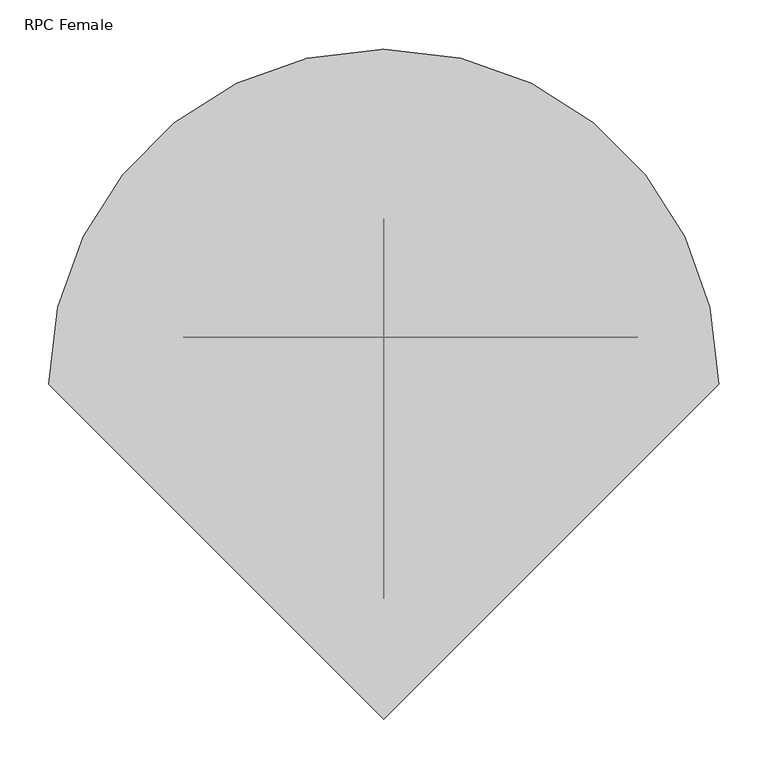
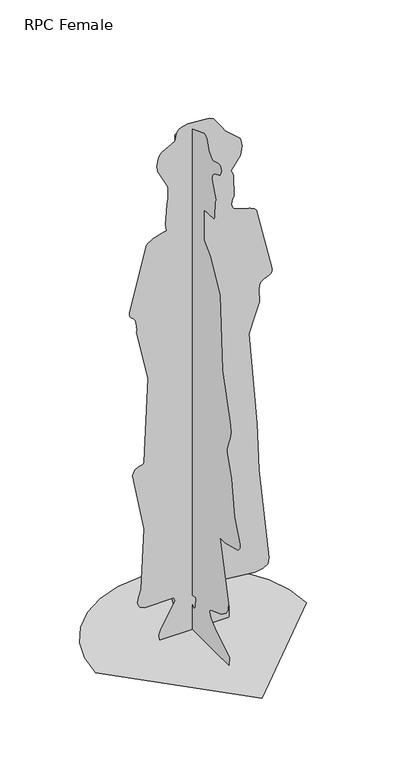
"""IFC4 building model written with IfcOpenShell, lengths in millimetres: proxy geometry, RPC Female : Tina."""

from ifc_helpers import new_model, si_unit, origin, place, context, project, spatial, triangles, source, transform, mapped, element, save


def rpc_female_936a91ee(model_context):
    return source(origin(), model_context, "Body", "Tessellation", [
        triangles([(119.4746024, 47.9851797, 38.3657269), (83.0886148, 47.9851797, 124.5051729), (83.0138374, 47.9851797, 136.8061299), (203.3585538, 47.9851751, 124.5967734), (228.5680434, 47.9851706, 128.329131), (244.5854705, 47.9851706, 139.121441), (247.7915793, 47.9851706, 159.148825), (216.0390116, 47.9851751, 471.099733), (209.7903923, 47.9851751, 633.4228918), (183.5555111, 47.9851751, 949.5239462), (203.8698598, 47.9851751, 1005.6493721), (217.070017, 47.9851751, 1047.2735756), (217.4083866, 47.9851706, 1056.0226055), (217.0055224, 47.9851751, 1064.6613224), (216.3185004, 47.9851751, 1073.2607248), (215.8053413, 47.9851751, 1081.8947908), (215.9203052, 47.9851751, 1090.6344463), (217.1204863, 47.9851751, 1099.5507626), (219.8629788, 47.9851706, 1108.7167002), (224.4103938, 47.9851706, 1115.2149227), (231.1179786, 47.9851706, 1119.4220787), (238.8976818, 47.9851706, 1122.5300285), (246.6605618, 47.9851706, 1125.7305599), (253.3176591, 47.9851706, 1130.2172047), (257.7819034, 47.9851706, 1137.1818232), (258.9624636, 47.9851706, 1147.8162031), (208.6911498, 47.9851751, 1362.8652134), (200.9254719, 47.9851751, 1370.8879795), (188.863799, 47.9851751, 1376.7655277), (174.3222992, 47.9851751, 1381.3783276), (159.1180856, 47.9851751, 1385.6033604), (145.0682618, 47.9851751, 1390.3226944), (133.9899228, 47.9851751, 1396.4143284), (127.6992275, 47.9851797, 1404.7577145), (126.3541607, 47.9851797, 1411.5830246), (128.3497965, 47.9851797, 1423.820359), (130.6183717, 47.9851751, 1429.1203262), (133.0196786, 47.9851751, 1433.7985291), (135.0181213, 47.9851751, 1437.799157), (133.6702475, 47.9851751, 1508.2801746), (130.0547342, 47.9851797, 1519.8473465), (124.9062748, 47.9851797, 1527.6429462), (155.2875963, 47.9851751, 1570.9468437), (160.9333272, 47.9851751, 1602.216156), (158.4198542, 47.9851751, 1619.8076694), (154.1621926, 47.9851751, 1629.1810799), (105.3565325, 47.9851797, 1672.8710003), (96.1467022, 47.9851797, 1688.204076), (68.7667873, 47.9851797, 1725.4903175), (55.188996, 47.9851797, 1733.4578545), (-13.8945541, 47.9851842, 1738.3893848), (-32.3179538, 47.9851842, 1734.7964355), (-43.8552446, 47.9851888, 1729.3150841), (-50.2795981, 47.9851888, 1722.1411034), (-56.6291742, 47.9851888, 1692.4206791), (-98.9749634, 47.9851888, 1670.8593498), (-105.122635, 47.9851888, 1663.7452492), (-109.692496, 47.9851888, 1653.3211761), (-114.0595259, 47.9851888, 1629.2249725), (-112.6097689, 47.9851888, 1608.9376934), (-83.4211617, 47.9851888, 1552.7197586), (-78.9718784, 47.9851888, 1541.6076462), (-78.7961533, 47.9851888, 1505.3964844), (-81.7470724, 47.9851888, 1484.4297409), (-87.7106074, 47.9851888, 1417.742823), (-84.5577838, 47.9851888, 1396.3797375), (-94.0555144, 47.9851888, 1393.929887), (-104.4290727, 47.9851888, 1391.1480801), (-115.0886601, 47.9851888, 1387.9241489), (-125.443524, 47.9851888, 1384.1517048), (-134.9057281, 47.9851933, 1379.7201439), (-142.8845289, 47.9851933, 1374.5230774), (-148.7929164, 47.9851933, 1368.4510643), (-204.6501356, 47.9851933, 1156.1950521), (-204.1388296, 47.9851933, 1148.5901384), (-202.0413195, 47.9851933, 1142.7341005), (-198.8511073, 47.9851933, 1138.1399042), (-195.0664001, 47.9851933, 1134.3234221), (-191.1816989, 47.9851933, 1130.7976925), (-187.6942483, 47.9851933, 1127.0793148), (-185.0994576, 47.9851933, 1122.6805281), (-182.0700095, 47.9851933, 1112.4219246), (-180.6408271, 47.9851933, 1101.7427073), (-180.2996415, 47.9851933, 1090.7111132), (-180.530514, 47.9851933, 1079.4000303), (-143.207011, 47.9851933, 910.4244432), (-157.1708389, 47.9851933, 628.3473295), (-159.6740291, 47.9851933, 622.3323624), (-164.457022, 47.9851933, 619.3833418), (-170.6897448, 47.9851933, 617.905525), (-177.5403441, 47.9851933, 616.306204), (-184.1759492, 47.9851933, 612.9907814), (-189.7665237, 47.9851933, 606.3635696), (-193.4783066, 47.9851933, 594.8328054), (-157.1708389, 47.9851933, 399.3335103), (-167.0209644, 47.9851933, 194.3290177), (-169.4288116, 47.9851933, 186.8839417), (-172.2367252, 47.9851933, 178.8920603), (-174.9072199, 47.9851933, 170.540299), (-176.9037914, 47.9851933, 162.0137664), (-177.6871011, 47.9851933, 153.5002962), (-176.7215169, 47.9851933, 145.1849971), (-169.586778, 47.9851933, 134.8759334), (-155.7790452, 47.9851933, 128.7095583), (-59.4221315, 47.9851888, 128.4272718), (-56.6291742, 47.9851888, 117.2563875), (-101.8137164, 47.9851888, 37.3721147), (-107.4482289, 47.9851888, 18.1869156), (-106.579868, 47.9851888, 0.0), (119.1848399, 47.9851797, 0.0), (0.0001119, 54.9526141, 116.0094705), (0.0001121, 60.1094851, 113.0529377), (0.0001122, 62.0593161, 108.0970356), (0.0001121, 60.01788, 100.4276273), (0.0001118, 53.2028118, 89.327787), (0.0001113, 44.8622735, 80.334813), (0.000111, 38.3650093, 77.9905248), (0.0001108, 33.5539884, 80.9825751), (0.0001106, 30.274978, 87.997672), (0.0001105, 28.0671617, 120.0493493), (0.0001166, 146.2769726, 6.9178889), (0.0001175, 162.7374504, 35.3007682), (0.0001176, 164.9162963, 41.8494396), (0.0001177, 166.2651057, 56.8797948), (0.0001176, 163.8385642, 70.5482556), (0.0001168, 149.0774012, 107.8250319), (0.0001167, 146.7153543, 120.4896022), (0.0001167, 148.1595067, 134.0131772), (0.0001174, 160.6203013, 134.9114508), (0.0001177, 167.0175489, 142.2088343), (0.0001178, 168.8972852, 153.9601882), (0.0001175, 162.8711087, 196.5003787), (0.0001174, 159.9987186, 373.2238758), (0.0001161, 135.8445243, 608.8527346), (0.0001162, 138.4767038, 634.7445408), (0.0001172, 157.6198485, 729.5666599), (0.0001172, 157.278663, 761.1135715), (0.000115, 115.0478559, 910.0384203), (0.0001159, 131.402717, 1267.9085094), (0.0001161, 136.0062332, 1279.6823547), (0.0001161, 135.2509741, 1291.9449783), (0.0001151, 116.6901702, 1339.5252136), (0.0001152, 117.680971, 1349.4584736), (0.0001158, 130.4455625, 1356.019265), (0.0001164, 141.4911909, 1365.0674046), (0.0001168, 149.9999739, 1376.6757076), (0.0001171, 155.1503045, 1390.9190243), (0.0001172, 156.1233556, 1407.8684258), (0.000117, 152.1002999, 1427.5975994), (0.0001149, 111.852039, 1516.4721165), (0.0001159, 131.1129545, 1509.7550846), (0.0001163, 139.0767943, 1509.2167454), (0.0001166, 146.2208895, 1510.6599712), (0.000117, 152.7630229, 1514.1615017), (0.0001173, 158.921913, 1519.7969135), (0.0001176, 164.9162963, 1527.6429462), (0.0001149, 111.852039, 1566.7424492), (0.0001151, 116.2414967, 1577.1785854), (0.0001165, 143.5849676, 1613.5468597), (0.0001167, 146.5237417, 1624.17281), (0.0001166, 145.366554, 1636.5634781), (0.0001134, 83.924365, 1700.7995281), (0.0001081, -16.6182319, 1739.8990311), (0.0001076, -26.3010313, 1738.9727795), (0.0001073, -33.3890412, 1728.6478283), (0.0001066, -46.2424218, 1696.3960178), (0.0001061, -55.2382026, 1682.7677799), (0.0001054, -68.0981281, 1676.3359051), (0.000104, -96.2931322, 1685.1905972), (0.0001035, -104.4298993, 1685.5785095), (0.0001032, -110.4663405, 1682.8799824), (0.000103, -114.0229639, 1677.5595222), (0.000103, -114.7165262, 1670.0845425), (0.0001031, -112.1656735, 1660.9186775), (0.0001035, -105.9899513, 1650.528178), (0.0001036, -103.0278138, 1647.7988388), (0.0001051, -75.2683935, 1636.5634781), (0.0001055, -66.247378, 1626.4553741), (0.0001057, -62.8907833, 1613.8730026), (0.0001057, -63.8451355, 1599.850312), (0.0001046, -83.6463206, 1549.9856232), (0.0001049, -78.0688267, 1540.9749813), (0.000105, -76.0376689, 1487.2693932), (0.0001052, -72.3529919, 1480.2656055), (0.0001081, -16.6182319, 1477.3715961), (0.0001081, -16.6182319, 1376.8290413), (0.000108, -18.9868203, 1370.1887489), (0.0001062, -52.9256984, 1337.7295383), (0.0001035, -106.1366992, 1240.4529179), (0.0001027, -121.4390628, 990.1572945), (0.0001003, -167.4321311, 829.4315672), (0.0001002, -168.6472641, 807.1813992), (0.0001003, -165.9197416, 788.9487185), (0.0001014, -145.2660968, 736.338703), (0.0001014, -145.0894361, 723.3030888), (0.0001, -173.0180366, 650.6890617), (9.92e-05, -188.1727075, 529.732128), (9.76e-05, -218.6998412, 452.8305356), (9.76e-05, -218.9812012, 439.9902583), (9.81e-05, -209.3245777, 427.2621108), (0.0001019, -135.0860223, 407.8011621), (0.0001035, -105.9890157, 407.7123957), (0.000101, -153.9291218, 211.1297364), (0.000101, -153.1813295, 187.819604), (0.0001016, -142.0497143, 170.5225493), (0.0001029, -116.6579502, 151.6738452), (0.000106, -57.8002783, 129.2423474), (0.0001064, -50.1327412, 128.4272718), (0.0001065, -47.3397885, 117.2563875), (0.000106, -57.0506329, 99.6892003), (0.0001045, -86.7954016, 72.5766065), (0.0001007, -158.9906406, 32.3862999), (0.0001006, -160.6077112, 29.508287), (0.0001006, -160.6591252, 24.7047421), (0.0001007, -159.8029275, 18.7813993), (0.0001007, -158.6924757, 12.5430548), (0.0001007, -157.9858146, 6.7963744), (0.0001007, -158.3382095, 2.3470907), (0.0001006, -160.4067424, 0.0), (0.0001165, 143.9840984, 0.0), (341.8443958, 0.0002001, 0.0), (332.8074838, 78.3281586, 0.0), (307.0689385, 150.2598054, 0.0), (266.6916975, 213.7350098, 0.0), (213.7349371, 266.6917701, 0.0), (150.2597327, 307.0690475, 0.0), (78.3280859, 332.8075928, 0.0), (0.0001269, 341.8445048, 0.0), (-78.3278316, 332.8075928, 0.0), (-150.2594784, 307.0690475, 0.0), (-213.7346828, 266.6918065, 0.0), (-266.6914431, 213.7350461, 0.0), (-307.0687205, 150.2598418, 0.0), (-332.8072658, 78.328195, 0.0), (-341.8441778, 0.0002359, 0.0), (9.11e-05, -341.8440688, 0.0)], [[108, 109, 110], [107, 108, 110], [107, 110, 1], [106, 107, 1], [106, 1, 2], [106, 2, 3], [105, 106, 3], [5, 6, 7], [4, 5, 7], [4, 7, 8], [3, 4, 8], [105, 3, 8], [104, 105, 8], [103, 104, 8], [102, 103, 8], [101, 102, 8], [100, 101, 8], [99, 100, 8], [98, 99, 8], [97, 98, 8], [96, 97, 8], [95, 96, 8], [95, 8, 9], [94, 95, 9], [93, 94, 9], [92, 93, 9], [91, 92, 9], [90, 91, 9], [89, 90, 9], [88, 89, 9], [87, 88, 9], [86, 87, 9], [86, 9, 10], [86, 10, 11], [85, 86, 11], [84, 85, 11], [84, 11, 12], [84, 12, 13], [84, 13, 14], [84, 14, 15], [84, 15, 16], [84, 16, 17], [83, 84, 17], [83, 17, 18], [82, 83, 18], [82, 18, 19], [81, 82, 19], [80, 81, 19], [80, 19, 20], [79, 80, 20], [78, 79, 20], [77, 78, 20], [76, 77, 20], [75, 76, 20], [74, 75, 20], [73, 74, 20], [72, 73, 20], [71, 72, 20], [70, 71, 20], [69, 70, 20], [68, 69, 20], [67, 68, 20], [66, 67, 20], [66, 20, 21], [66, 21, 22], [66, 22, 23], [66, 23, 24], [66, 24, 25], [66, 25, 26], [66, 26, 27], [66, 27, 28], [66, 28, 29], [66, 29, 30], [66, 30, 31], [66, 31, 32], [66, 32, 33], [66, 33, 34], [66, 34, 35], [65, 66, 35], [64, 65, 35], [64, 35, 36], [64, 36, 37], [63, 64, 37], [63, 37, 38], [63, 38, 39], [63, 39, 40], [63, 40, 41], [63, 41, 42], [62, 63, 42], [61, 62, 42], [61, 42, 43], [61, 43, 44], [61, 44, 45], [61, 45, 46], [61, 46, 47], [61, 47, 48], [60, 61, 48], [59, 60, 48], [58, 59, 48], [57, 58, 48], [56, 57, 48], [55, 56, 48], [55, 48, 49], [55, 49, 50], [55, 50, 51], [55, 51, 52], [55, 52, 53], [55, 53, 54], [218, 219, 220], [115, 123, 124], [115, 124, 125], [114, 115, 125], [114, 125, 126], [113, 114, 126], [113, 126, 127], [217, 218, 220], [155, 156, 157], [122, 123, 115], [122, 115, 116], [121, 122, 116], [216, 217, 220], [215, 216, 220], [214, 215, 220], [213, 214, 220], [212, 213, 220], [211, 212, 220], [210, 211, 220], [210, 220, 121], [209, 210, 121], [112, 113, 127], [112, 127, 128], [183, 184, 185], [180, 181, 182], [121, 116, 117], [209, 121, 117], [209, 117, 118], [209, 118, 119], [209, 119, 120], [208, 209, 120], [154, 155, 157], [153, 154, 157], [152, 153, 157], [151, 152, 157], [150, 151, 157], [163, 164, 165], [162, 163, 165], [162, 165, 166], [128, 129, 130], [128, 130, 131], [112, 128, 131], [112, 131, 132], [111, 112, 132], [120, 111, 132], [208, 120, 132], [208, 132, 133], [207, 208, 133], [206, 207, 133], [205, 206, 133], [204, 205, 133], [203, 204, 133], [202, 203, 133], [202, 133, 134], [182, 183, 185], [202, 134, 135], [180, 182, 185], [162, 166, 167], [161, 162, 167], [160, 161, 167], [159, 160, 167], [158, 159, 167], [157, 158, 167], [157, 167, 168], [150, 157, 168], [201, 202, 135], [200, 201, 135], [199, 200, 135], [198, 199, 135], [197, 198, 135], [196, 197, 135], [195, 196, 135], [195, 135, 136], [194, 195, 136], [194, 136, 137], [193, 194, 137], [192, 193, 137], [191, 192, 137], [191, 137, 138], [190, 191, 138], [190, 138, 139], [189, 190, 139], [188, 189, 139], [188, 139, 140], [188, 140, 141], [188, 141, 142], [187, 188, 142], [187, 142, 143], [186, 187, 143], [185, 186, 143], [185, 143, 144], [185, 144, 145], [185, 145, 146], [185, 146, 147], [185, 147, 148], [185, 148, 149], [185, 149, 150], [185, 150, 168], [170, 171, 172], [170, 172, 173], [169, 170, 173], [169, 173, 174], [169, 174, 175], [169, 175, 176], [168, 169, 176], [168, 176, 177], [168, 177, 178], [185, 168, 178], [185, 178, 179], [180, 185, 179], [235, 236, 221], [234, 235, 221], [234, 221, 222], [233, 234, 222], [233, 222, 223], [233, 223, 224], [232, 233, 224], [231, 232, 224], [231, 224, 225], [231, 225, 226], [231, 226, 227], [231, 227, 228], [231, 228, 229], [231, 229, 230]], closed=False),
    ])


if __name__ == "__main__":
    model = new_model("IFC4")
    model_context = context("Model", 3, world=origin())
    ifc_project = project(units=[si_unit("LENGTHUNIT", "METRE", prefix="MILLI")], contexts=[model_context])
    site = spatial("IfcSite", under=ifc_project)
    building = spatial("IfcBuilding", under=site)
    placement = place(None, origin())
    rpc_female_shape = rpc_female_936a91ee(model_context)
    element("IfcBuildingElementProxy", 1, Name="RPC Female : Tina", ObjectType="RPC Female : Tina", at=placement, inside=building, context=model_context, shape_type="MappedRepresentation", body=[
        mapped(rpc_female_shape, transform((0.0, 0.0, 0.0), x_axis=(1.0, 0.0, 0.0), y_axis=(0.0, 1.0, 0.0), z_axis=(0.0, 0.0, 1.0))),
    ])
    save(model, "model.ifc")

# Revit data of these elements
# Type "RPC Female : Tina"
#   built-in parameter 1005198 = "{2, 15},{22, RPC-8-E23G-6DS7-USQ4-G},{1, 0},{1, 0},{2, 15},{1, 8},{5, Color},{1, 0},{1, 0},{3, 0.8},{3, 0.8},{3, 0.8},{1, 8},{7, BBoxMin},{1, 0},{1, 0},{1, 0},{1, 0},{1, 0},{1, 8},{7, BBoxMax},{1, 0},{1, 0},{1, 0},{1, 0},{1, 0},{2, 11},{9, RPCTypeId},{1, 0},{1, 0},{22, RPC-8-E23G-6DS7-USQ4-G},{1, 6},{14, RPCPlantHeight},{1, 0},{1, 0},{7, 5.70833},{2, 11},{7, keyword},{1, 0},{1, 0},{34, :RPCs:People [Casual]:Geometry:RPC},{2, 11},{8, category},{1, 0},{1, 0},{15, People [Casual]},{2, 11},{12, LocalizedUID},{1, 0},{1, 0},{8, Tina [2]},{2, 14},{6, Height},{1, 0},{1, 0},{7, 5.70833},{1, 2},{16, Cast Reflections},{1, 0},{1, 0},{1, 0},{1, 2},{6, Jitter},{1, 0},{1, 0},{1, 1},{1, 2},{9, Billboard},{1, 0},{1, 0},{1, 0},{1, 2},{12, Cast Shadows},{1, 0},{1, 0},{1, 1},{1, 2},{20, Apply Filter Effects},{1, 0},{1, 0},{1, 0},{2, 11},{28, Apply Filter Effects-Text-FC},{1, 0},{1, 0},{4, None},{21, assetlibrary_base.fbx},{1, 5},"
#   built-in parameter 1005195 = "RPC-8-E23G-6DS7-USQ4-G"
#   Height = 0
